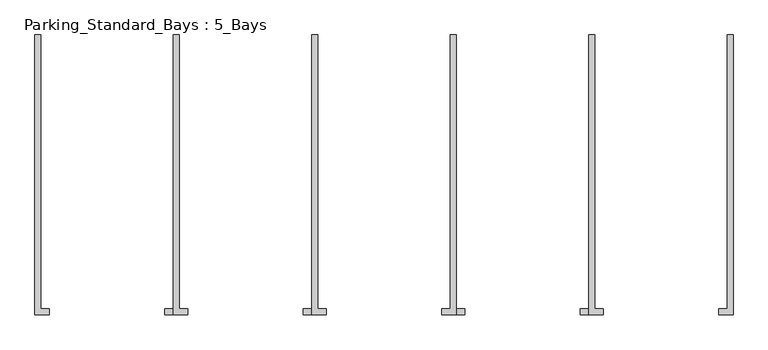
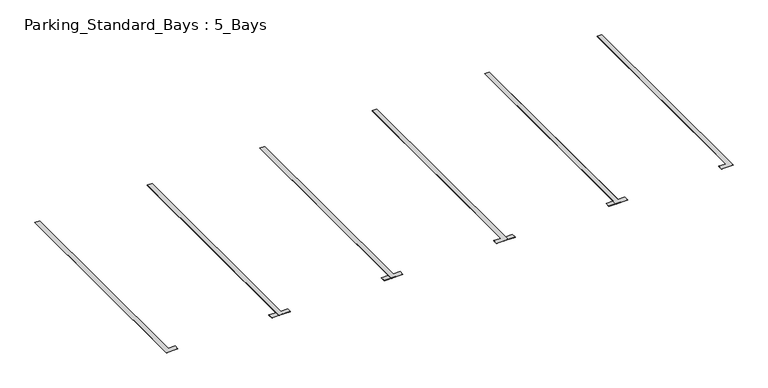
"""IFC4 building model written with IfcOpenShell, lengths in millimetres: proxy geometry, Parking_Standard_Bays : 5_Bays."""

from ifc_helpers import new_model, si_unit, origin, origin_with_axes, place, context, project, spatial, polyline, outline, extrude, source, transform, mapped, element, save


def parking_standard_bays_5_bays_6c4ea7f3(model_context):
    return source(origin(), model_context, "Body", "SweptSolid", [
        extrude(outline(polyline([(11950.0, 0.0), (12050.0, 0.0), (12050.0, -4850.0), (11800.0, -4850.0), (11800.0, -4750.0), (11950.0, -4750.0), (11950.0, 0.0)])), origin_with_axes(), (0.0, 0.0, 1.0), 3.175),
        extrude(outline(polyline([(9550.0, 0.0), (9650.0, 0.0), (9650.0, -4750.0), (9800.0, -4750.0), (9800.0, -4850.0), (9550.0, -4850.0), (9550.0, 0.0)])), origin_with_axes(), (0.0, 0.0, 1.0), 3.175),
        extrude(outline(polyline([(7150.0, 0.0), (7250.0, 0.0), (7250.0, -4850.0), (7000.0, -4850.0), (7000.0, -4750.0), (7150.0, -4750.0), (7150.0, 0.0)])), origin_with_axes(), (0.0, 0.0, 1.0), 3.175),
        extrude(outline(polyline([(4750.0, 0.0), (4850.0, 0.0), (4850.0, -4750.0), (5000.0, -4750.0), (5000.0, -4850.0), (4750.0, -4850.0), (4750.0, 0.0)])), origin_with_axes(), (0.0, 0.0, 1.0), 3.175),
        extrude(outline(polyline([(4750.0, 0.0), (4850.0, 0.0), (4850.0, -4850.0), (4600.0, -4850.0), (4600.0, -4750.0), (4750.0, -4750.0), (4750.0, 0.0)])), origin_with_axes(), (0.0, 0.0, 1.0), 3.175),
        extrude(outline(polyline([(2350.0, 0.0), (2450.0, 0.0), (2450.0, -4750.0), (2600.0, -4750.0), (2600.0, -4850.0), (2350.0, -4850.0), (2350.0, 0.0)])), origin_with_axes(), (0.0, 0.0, 1.0), 3.175),
        extrude(outline(polyline([(9550.0, 0.0), (9650.0, 0.0), (9650.0, -4850.0), (9400.0, -4850.0), (9400.0, -4750.0), (9550.0, -4750.0), (9550.0, 0.0)])), origin_with_axes(), (0.0, 0.0, 1.0), 3.175),
        extrude(outline(polyline([(7150.0, 0.0), (7250.0, 0.0), (7250.0, -4750.0), (7400.0, -4750.0), (7400.0, -4850.0), (7150.0, -4850.0), (7150.0, 0.0)])), origin_with_axes(), (0.0, 0.0, 1.0), 3.175),
        extrude(outline(polyline([(2350.0, 0.0), (2450.0, 0.0), (2450.0, -4850.0), (2200.0, -4850.0), (2200.0, -4750.0), (2350.0, -4750.0), (2350.0, 0.0)])), origin_with_axes(), (0.0, 0.0, 1.0), 3.175),
        extrude(outline(polyline([(-50.0, 0.0), (50.0, 0.0), (50.0, -4750.0), (200.0, -4750.0), (200.0, -4850.0), (-50.0, -4850.0), (-50.0, 0.0)])), origin_with_axes(), (0.0, 0.0, 1.0), 3.175),
    ])


if __name__ == "__main__":
    model = new_model("IFC4")
    model_context = context("Model", 3, world=origin())
    ifc_project = project(units=[si_unit("LENGTHUNIT", "METRE", prefix="MILLI")], contexts=[model_context])
    site = spatial("IfcSite", under=ifc_project)
    building = spatial("IfcBuilding", under=site)
    placement = place(None, origin())
    parking_standard_bays_5_bays_shape = parking_standard_bays_5_bays_6c4ea7f3(model_context)
    element("IfcBuildingElementProxy", 1, Name="Parking_Standard_Bays : 5_Bays", ObjectType="Parking_Standard_Bays : 5_Bays", at=placement, inside=building, context=model_context, shape_type="MappedRepresentation", body=[
        mapped(parking_standard_bays_5_bays_shape, transform((0.0, 0.0, 0.0), x_axis=(1.0, 0.0, 0.0), y_axis=(0.0, 1.0, 0.0), z_axis=(0.0, 0.0, 1.0))),
    ])
    save(model, "model.ifc")

# Revit data of these elements
# Type "Parking_Standard_Bays : 5_Bays"
#   Keynote = "Q22/185"
#   Length [instance default] = 14400 mm
#   Bay Width = 2400 mm
#   Bay Length = 4800 mm
#   No of Bays in Array [instance default] = 5
#   No of Bays [instance default] = 6
#   Material - White Lining = Paint - White Lining
# Element 1 (IfcBuildingElementProxy, "Parking_Standard_Bays : 5_Bays")
#   Length = 12000 mm
#   No of Bays in Array = 4
#   No of Bays = 5
#   Materials on its faces: "Paint - White Lining"
# Materials
#   "Paint - White Lining": class "Paint", colour RGB 239 247 247, transparency 0
